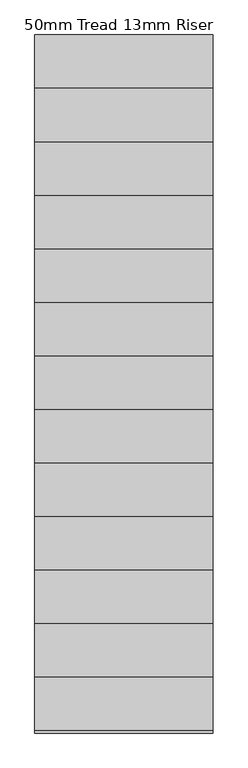
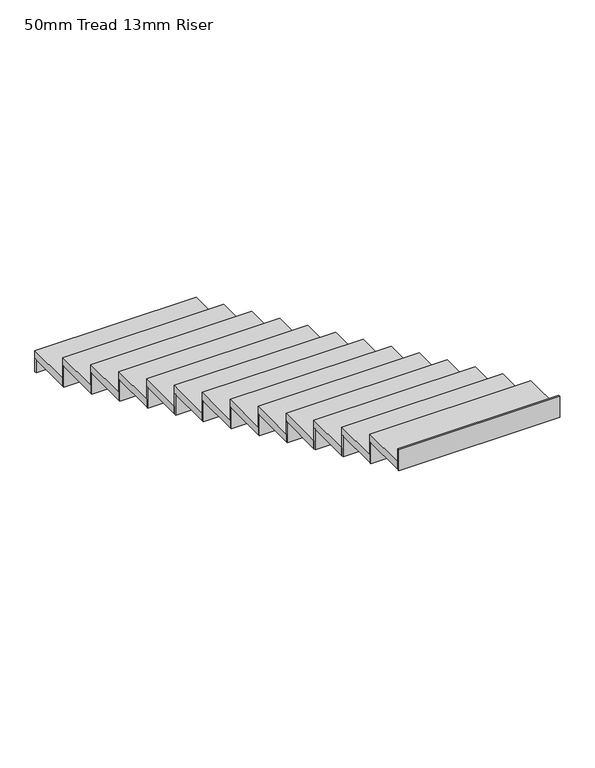
"""IFC4 building model written with IfcOpenShell, lengths in millimetres: stair flight geometry, 50mm Tread 13mm Riser."""

from ifc_helpers import new_model, si_unit, frame, origin, origin_with_axes, place, context, project, spatial, polyline, outline, extrude, source, transform, mapped, element, save


def stair_flight_50mm_tread_13mm_riser_9427a4d1(model_context):
    return source(origin(), model_context, "Body", "SweptSolid", [
        extrude(outline(polyline([(-13626.101437, 1647.3621849), (-13626.101437, 1659.8621849), (-12626.101437, 1659.8621849), (-12626.101437, 1647.3621849), (-13626.101437, 1647.3621849)])), origin_with_axes(), (0.0, 0.0, 1.0), 86.3636364),
        extrude(outline(polyline([(-12626.101437, 1359.8621849), (-13626.101437, 1359.8621849), (-13626.101437, 1659.8621849), (-12626.101437, 1659.8621849), (-12626.101437, 1359.8621849)])), frame((0.0, 0.0, 86.3636364), z_axis=(0.0, 0.0, 1.0), x_axis=(1.0, 0.0, 0.0)), (0.0, 0.0, 1.0), 50.0),
        extrude(outline(polyline([(-13626.101437, 1347.3621849), (-13626.101437, 1359.8621849), (-12626.101437, 1359.8621849), (-12626.101437, 1347.3621849), (-13626.101437, 1347.3621849)])), frame((0.0, 0.0, 86.3636364), z_axis=(0.0, 0.0, 1.0), x_axis=(1.0, 0.0, 0.0)), (0.0, 0.0, 1.0), 136.3636364),
        extrude(outline(polyline([(-12626.101437, 1059.8621849), (-13626.101437, 1059.8621849), (-13626.101437, 1359.8621849), (-12626.101437, 1359.8621849), (-12626.101437, 1059.8621849)])), frame((0.0, 0.0, 222.7272727), z_axis=(0.0, 0.0, 1.0), x_axis=(1.0, 0.0, 0.0)), (0.0, 0.0, 1.0), 50.0),
        extrude(outline(polyline([(-13626.101437, 1047.3621849), (-13626.101437, 1059.8621849), (-12626.101437, 1059.8621849), (-12626.101437, 1047.3621849), (-13626.101437, 1047.3621849)])), frame((0.0, 0.0, 222.7272727), z_axis=(0.0, 0.0, 1.0), x_axis=(1.0, 0.0, 0.0)), (0.0, 0.0, 1.0), 136.3636364),
        extrude(outline(polyline([(-12626.101437, 759.8621849), (-13626.101437, 759.8621849), (-13626.101437, 1059.8621849), (-12626.101437, 1059.8621849), (-12626.101437, 759.8621849)])), frame((0.0, 0.0, 359.0909091), z_axis=(0.0, 0.0, 1.0), x_axis=(1.0, 0.0, 0.0)), (0.0, 0.0, 1.0), 50.0),
        extrude(outline(polyline([(-13626.101437, 747.3621849), (-13626.101437, 759.8621849), (-12626.101437, 759.8621849), (-12626.101437, 747.3621849), (-13626.101437, 747.3621849)])), frame((0.0, 0.0, 359.0909091), z_axis=(0.0, 0.0, 1.0), x_axis=(1.0, 0.0, 0.0)), (0.0, 0.0, 1.0), 136.3636364),
        extrude(outline(polyline([(-12626.101437, 459.8621849), (-13626.101437, 459.8621849), (-13626.101437, 759.8621849), (-12626.101437, 759.8621849), (-12626.101437, 459.8621849)])), frame((0.0, 0.0, 495.4545455), z_axis=(0.0, 0.0, 1.0), x_axis=(1.0, 0.0, 0.0)), (0.0, 0.0, 1.0), 50.0),
        extrude(outline(polyline([(-13626.101437, 447.3621849), (-13626.101437, 459.8621849), (-12626.101437, 459.8621849), (-12626.101437, 447.3621849), (-13626.101437, 447.3621849)])), frame((0.0, 0.0, 495.4545455), z_axis=(0.0, 0.0, 1.0), x_axis=(1.0, 0.0, 0.0)), (0.0, 0.0, 1.0), 136.3636364),
        extrude(outline(polyline([(-12626.101437, 159.8621849), (-13626.101437, 159.8621849), (-13626.101437, 459.8621849), (-12626.101437, 459.8621849), (-12626.101437, 159.8621849)])), frame((0.0, 0.0, 631.8181818), z_axis=(0.0, 0.0, 1.0), x_axis=(1.0, 0.0, 0.0)), (0.0, 0.0, 1.0), 50.0),
        extrude(outline(polyline([(-13626.101437, 147.3621849), (-13626.101437, 159.8621849), (-12626.101437, 159.8621849), (-12626.101437, 147.3621849), (-13626.101437, 147.3621849)])), frame((0.0, 0.0, 631.8181818), z_axis=(0.0, 0.0, 1.0), x_axis=(1.0, 0.0, 0.0)), (0.0, 0.0, 1.0), 136.3636364),
        extrude(outline(polyline([(-12626.101437, -140.1378151), (-13626.101437, -140.1378151), (-13626.101437, 159.8621849), (-12626.101437, 159.8621849), (-12626.101437, -140.1378151)])), frame((0.0, 0.0, 768.1818182), z_axis=(0.0, 0.0, 1.0), x_axis=(1.0, 0.0, 0.0)), (0.0, 0.0, 1.0), 50.0),
        extrude(outline(polyline([(-13626.101437, -152.6378151), (-13626.101437, -140.1378151), (-12626.101437, -140.1378151), (-12626.101437, -152.6378151), (-13626.101437, -152.6378151)])), frame((0.0, 0.0, 768.1818182), z_axis=(0.0, 0.0, 1.0), x_axis=(1.0, 0.0, 0.0)), (0.0, 0.0, 1.0), 136.3636364),
        extrude(outline(polyline([(-12626.101437, -440.1378151), (-13626.101437, -440.1378151), (-13626.101437, -140.1378151), (-12626.101437, -140.1378151), (-12626.101437, -440.1378151)])), frame((0.0, 0.0, 904.5454545), z_axis=(0.0, 0.0, 1.0), x_axis=(1.0, 0.0, 0.0)), (0.0, 0.0, 1.0), 50.0),
        extrude(outline(polyline([(-13626.101437, -452.6378151), (-13626.101437, -440.1378151), (-12626.101437, -440.1378151), (-12626.101437, -452.6378151), (-13626.101437, -452.6378151)])), frame((0.0, 0.0, 904.5454545), z_axis=(0.0, 0.0, 1.0), x_axis=(1.0, 0.0, 0.0)), (0.0, 0.0, 1.0), 136.3636364),
        extrude(outline(polyline([(-12626.101437, -740.1378151), (-13626.101437, -740.1378151), (-13626.101437, -440.1378151), (-12626.101437, -440.1378151), (-12626.101437, -740.1378151)])), frame((0.0, 0.0, 1040.9090909), z_axis=(0.0, 0.0, 1.0), x_axis=(1.0, 0.0, 0.0)), (0.0, 0.0, 1.0), 50.0),
        extrude(outline(polyline([(-13626.101437, -752.6378151), (-13626.101437, -740.1378151), (-12626.101437, -740.1378151), (-12626.101437, -752.6378151), (-13626.101437, -752.6378151)])), frame((0.0, 0.0, 1040.9090909), z_axis=(0.0, 0.0, 1.0), x_axis=(1.0, 0.0, 0.0)), (0.0, 0.0, 1.0), 136.3636364),
        extrude(outline(polyline([(-12626.101437, -1040.1378151), (-13626.101437, -1040.1378151), (-13626.101437, -740.1378151), (-12626.101437, -740.1378151), (-12626.101437, -1040.1378151)])), frame((0.0, 0.0, 1177.2727273), z_axis=(0.0, 0.0, 1.0), x_axis=(1.0, 0.0, 0.0)), (0.0, 0.0, 1.0), 50.0),
        extrude(outline(polyline([(-13626.101437, -1052.6378151), (-13626.101437, -1040.1378151), (-12626.101437, -1040.1378151), (-12626.101437, -1052.6378151), (-13626.101437, -1052.6378151)])), frame((0.0, 0.0, 1177.2727273), z_axis=(0.0, 0.0, 1.0), x_axis=(1.0, 0.0, 0.0)), (0.0, 0.0, 1.0), 136.3636364),
        extrude(outline(polyline([(-12626.101437, -1340.1378151), (-13626.101437, -1340.1378151), (-13626.101437, -1040.1378151), (-12626.101437, -1040.1378151), (-12626.101437, -1340.1378151)])), frame((0.0, 0.0, 1313.6363636), z_axis=(0.0, 0.0, 1.0), x_axis=(1.0, 0.0, 0.0)), (0.0, 0.0, 1.0), 50.0),
        extrude(outline(polyline([(-13626.101437, -1352.6378151), (-13626.101437, -1340.1378151), (-12626.101437, -1340.1378151), (-12626.101437, -1352.6378151), (-13626.101437, -1352.6378151)])), frame((0.0, 0.0, 1313.6363636), z_axis=(0.0, 0.0, 1.0), x_axis=(1.0, 0.0, 0.0)), (0.0, 0.0, 1.0), 136.3636364),
        extrude(outline(polyline([(-12626.101437, -1640.1378151), (-13626.101437, -1640.1378151), (-13626.101437, -1340.1378151), (-12626.101437, -1340.1378151), (-12626.101437, -1640.1378151)])), frame((0.0, 0.0, 1450.0), z_axis=(0.0, 0.0, 1.0), x_axis=(1.0, 0.0, 0.0)), (0.0, 0.0, 1.0), 50.0),
        extrude(outline(polyline([(-13626.101437, -1652.6378151), (-13626.101437, -1640.1378151), (-12626.101437, -1640.1378151), (-12626.101437, -1652.6378151), (-13626.101437, -1652.6378151)])), frame((0.0, 0.0, 1450.0), z_axis=(0.0, 0.0, 1.0), x_axis=(1.0, 0.0, 0.0)), (0.0, 0.0, 1.0), 136.3636364),
        extrude(outline(polyline([(-12626.101437, -1940.1378151), (-13626.101437, -1940.1378151), (-13626.101437, -1640.1378151), (-12626.101437, -1640.1378151), (-12626.101437, -1940.1378151)])), frame((0.0, 0.0, 1586.3636364), z_axis=(0.0, 0.0, 1.0), x_axis=(1.0, 0.0, 0.0)), (0.0, 0.0, 1.0), 50.0),
        extrude(outline(polyline([(-13626.101437, -1952.6378151), (-13626.101437, -1940.1378151), (-12626.101437, -1940.1378151), (-12626.101437, -1952.6378151), (-13626.101437, -1952.6378151)])), frame((0.0, 0.0, 1586.3636364), z_axis=(0.0, 0.0, 1.0), x_axis=(1.0, 0.0, 0.0)), (0.0, 0.0, 1.0), 136.3636364),
        extrude(outline(polyline([(-13626.101437, -2252.6378151), (-13626.101437, -2240.1378151), (-12626.101437, -2240.1378151), (-12626.101437, -2252.6378151), (-13626.101437, -2252.6378151)])), frame((0.0, 0.0, 1722.7272727), z_axis=(0.0, 0.0, 1.0), x_axis=(1.0, 0.0, 0.0)), (0.0, 0.0, 1.0), 136.3636364),
        extrude(outline(polyline([(-12626.101437, -2240.1378151), (-13626.101437, -2240.1378151), (-13626.101437, -1940.1378151), (-12626.101437, -1940.1378151), (-12626.101437, -2240.1378151)])), frame((0.0, 0.0, 1722.7272727), z_axis=(0.0, 0.0, 1.0), x_axis=(1.0, 0.0, 0.0)), (0.0, 0.0, 1.0), 50.0),
    ])


if __name__ == "__main__":
    model = new_model("IFC4")
    model_context = context("Model", 3, world=origin())
    ifc_project = project(units=[si_unit("LENGTHUNIT", "METRE", prefix="MILLI")], contexts=[model_context])
    site = spatial("IfcSite", under=ifc_project)
    building = spatial("IfcBuilding", under=site)
    placement = place(None, origin())
    stair_flight_50mm_tread_13mm_riser_shape = stair_flight_50mm_tread_13mm_riser_9427a4d1(model_context)
    element("IfcStairFlight", 1, ObjectType="50mm Tread 13mm Riser", at=placement, inside=building, context=model_context, shape_type="MappedRepresentation", body=[
        mapped(stair_flight_50mm_tread_13mm_riser_shape, transform((0.0, 0.0, 0.0), x_axis=(1.0, 0.0, 0.0), y_axis=(0.0, 1.0, 0.0), z_axis=(0.0, 0.0, 1.0))),
    ])
    save(model, "model.ifc")
